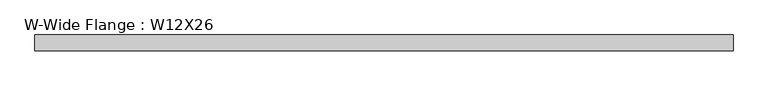
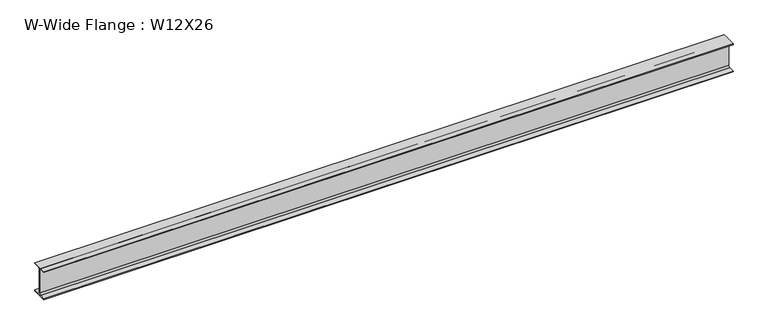
"""IFC4 building model written with IfcOpenShell, lengths in millimetres: beam geometry, W-Wide Flange : W12X26."""

from ifc_helpers import new_model, si_unit, point, frame, frame_2d, origin, place, context, project, spatial, polyline, circle_curve, trimmed, segment, composite_curve, outline, extrude, source, transform, mapped, element, save


def w_wide_flange_w12x26_06ae670e(model_context):
    return source(origin(), model_context, "Body", "SweptSolid", [
        extrude(outline(composite_curve([segment(polyline([(82.4011719, -145.5539063), (82.4011719, -155.178125), (-82.4011719, -155.178125), (-82.4011719, -145.5539063), (-20.2902344, -145.5539063)]), True, "CONTINUOUS"), segment(trimmed(circle_curve(frame_2d((-20.2902344, -128.190625)), 17.3632812), [point((-20.2902344, -145.5539063))], [point((-2.9269531, -128.190625))], True, "CARTESIAN"), True, "CONTINUOUS"), segment(polyline([(-2.9269531, -128.190625), (-2.9269531, 128.190625)]), True, "CONTINUOUS"), segment(trimmed(circle_curve(frame_2d((-20.2902344, 128.190625)), 17.3632812), [point((-2.9269531, 128.190625))], [point((-20.2902344, 145.5539062))], True, "CARTESIAN"), True, "CONTINUOUS"), segment(polyline([(-20.2902344, 145.5539062), (-82.4011719, 145.5539062), (-82.4011719, 155.178125), (82.4011719, 155.178125), (82.4011719, 145.5539062), (20.2902344, 145.5539062)]), True, "CONTINUOUS"), segment(trimmed(circle_curve(frame_2d((20.2902344, 128.190625)), 17.3632812), [point((20.2902344, 145.5539062))], [point((2.9269531, 128.190625))], True, "CARTESIAN"), True, "CONTINUOUS"), segment(polyline([(2.9269531, 128.190625), (2.9269531, -128.190625)]), True, "CONTINUOUS"), segment(trimmed(circle_curve(frame_2d((20.2902344, -128.190625)), 17.3632812), [point((2.9269531, -128.190625))], [point((20.2902344, -145.5539063))], True, "CARTESIAN"), True, "CONTINUOUS"), segment(polyline([(20.2902344, -145.5539063), (82.4011719, -145.5539063)]), True, "CONTINUOUS")], self_intersect=False)), frame((-3511.3132351, 0.0, 0.0), z_axis=(1.0, 0.0, 0.0), x_axis=(0.0, 1.0, 0.0)), (0.0, 0.0, 1.0), 7219.327642),
    ])


if __name__ == "__main__":
    model = new_model("IFC4")
    model_context = context("Model", 3, world=origin())
    ifc_project = project(units=[si_unit("LENGTHUNIT", "METRE", prefix="MILLI")], contexts=[model_context])
    site = spatial("IfcSite", under=ifc_project)
    building = spatial("IfcBuilding", under=site)
    placement = place(None, origin())
    w_wide_flange_w12x26_shape = w_wide_flange_w12x26_06ae670e(model_context)
    element("IfcBeam", 1, ObjectType="W-Wide Flange : W12X26", at=placement, inside=building, context=model_context, shape_type="MappedRepresentation", body=[
        mapped(w_wide_flange_w12x26_shape, transform((0.0, 0.0, 0.0), x_axis=(1.0, 0.0, 0.0), y_axis=(0.0, 1.0, 0.0), z_axis=(0.0, 0.0, 1.0))),
    ])
    save(model, "model.ifc")

# Revit data of these elements
# Type "W-Wide Flange : W12X26"
#   Assembly Code = "B10"
#   W = 26
#   Length [instance default] = 5' - 0"
#   bf = 0' - 6 125/256"
#   d = 1' - 0 7/32"
#   k = 0' - 1 1/16"
#   k2 = 0' - 0 175/256"
#   tf = 0' - 0 97/256"
#   tw = 0' - 0 59/256"
#   A = 0.053125 SF
#   Structural Material [instance default] = none
# Element 1 (IfcBeam, "W-Wide Flange : W12X26")
#   Structural Material = Dark metal
#   Materials on its faces: "Dark metal"
# Materials
#   "Dark metal": class "Generic", colour RGB 44 29 29, transparency 0, Cost = 0
